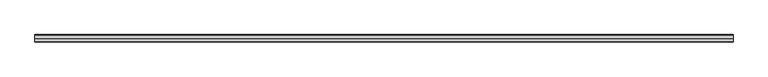
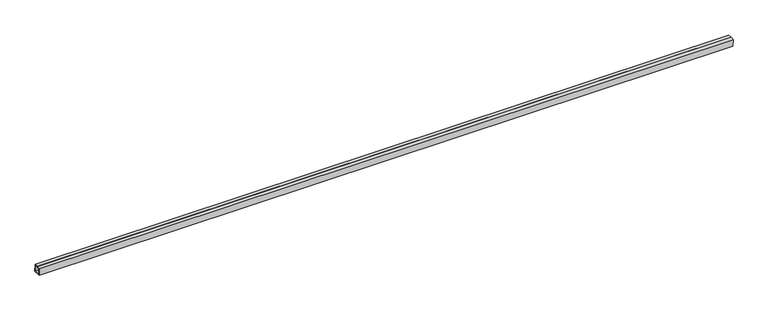
"""IFC4 building model written with IfcOpenShell, lengths in millimetres: proxy geometry, Inner panel:Inner panel:1:Inner panel:1 : Inner panel:Inner panel:300324:2:Inner panel:1:Inner panel:1 : Inner panel:Inner panel:300324:2 : Inner panel:Inner panel:1:Inner panel:1 : Inner panel:Inner panel:300324:300043:19 : Inner panel:Inner panel:1:Inner panel:1 : Inner panel:Inner panel:300324:2:Inner panel:1:Inner panel:1 : Inner panel:Inner panel:300324:2 : Inner panel:Inner panel:1:Inner panel:1 : Inner panel:Inner panel:300324:300043:308120."""

from ifc_helpers import new_model, si_unit, frame, origin, place, context, project, spatial, polyline, outline, extrude, source, transform, mapped, element, save


def generic_models_f3daa5ce(model_context):
    return source(origin(), model_context, "Body", "SweptSolid", [
        extrude(outline(polyline([(-569791.292732, 8736.8354816), (-569773.0523088, 8737.5954993), (-569771.4661851, 8699.5285292), (-569809.5331552, 8697.9424054), (-569811.1192789, 8736.0093755), (-569792.8788557, 8736.7693931), (-569792.779723, 8734.3902075), (-569808.6409605, 8733.7293226), (-569807.2531023, 8700.4207238), (-569773.9445034, 8701.8085821), (-569775.3323617, 8735.1171809), (-569791.1935993, 8734.456296), (-569791.292732, 8736.8354816)])), frame((593141.1867242, 0.0, 0.0), z_axis=(1.0, 0.0, 0.0), x_axis=(0.0, 1.0, 0.0)), (0.0, 0.0, 1.0), 3657.6),
    ])


if __name__ == "__main__":
    model = new_model("IFC4")
    model_context = context("Model", 3, world=origin())
    ifc_project = project(units=[si_unit("LENGTHUNIT", "METRE", prefix="MILLI")], contexts=[model_context])
    site = spatial("IfcSite", under=ifc_project)
    building = spatial("IfcBuilding", under=site)
    placement = place(None, origin())
    generic_models_shape = generic_models_f3daa5ce(model_context)
    element("IfcBuildingElementProxy", 1, Name="Inner panel:Inner panel:1:Inner panel:1 : Inner panel:Inner panel:300324:2:Inner panel:1:Inner panel:1 : Inner panel:Inner panel:300324:2 : Inner panel:Inner panel:1:Inner panel:1 : Inner panel:Inner panel:300324:300043:19 : Inner panel:Inner panel:1:Inner panel:1 : Inner panel:Inner panel:300324:2:Inner panel:1:Inner panel:1 : Inner panel:Inner panel:300324:2 : Inner panel:Inner panel:1:Inner panel:1 : Inner panel:Inner panel:300324:300043:308120", ObjectType="Inner panel:Inner panel:1:Inner panel:1 : Inner panel:Inner panel:300324:2:Inner panel:1:Inner panel:1 : Inner panel:Inner panel:300324:2 : Inner panel:Inner panel:1:Inner panel:1 : Inner panel:Inner panel:300324:300043:19 : Inner panel:Inner panel:1:Inner panel:1 : Inner panel:Inner panel:300324:2:Inner panel:1:Inner panel:1 : Inner panel:Inner panel:300324:2 : Inner panel:Inner panel:1:Inner panel:1 : Inner panel:Inner panel:300324:300043:308120", at=placement, inside=building, context=model_context, shape_type="MappedRepresentation", body=[
        mapped(generic_models_shape, transform((0.0, 0.0, 0.0), x_axis=(1.0, 0.0, 0.0), y_axis=(0.0, 1.0, 0.0), z_axis=(0.0, 0.0, 1.0))),
    ])
    save(model, "model.ifc")

# Revit data of these elements
# Type "Inner panel:Inner panel:1:Inner panel:1 : Inner panel:Inner panel:300324:2:Inner panel:1:Inner panel:1 : Inner panel:Inner panel:300324:2 : Inner panel:Inner panel:1:Inner panel:1 : Inner panel:Inner panel:300324:300043:19 : Inner panel:Inner panel:1:Inner panel:1 : Inner panel:Inner panel:300324:2:Inner panel:1:Inner panel:1 : Inner panel:Inner panel:300324:2 : Inner panel:Inner panel:1:Inner panel:1 : Inner panel:Inner panel:300324:300043:308120"
#   NameOverride = "Inner panel:Inner panel:1:Inner panel:1 : Inner panel:Inner panel:300324:2:Inner panel:1:Inner panel:1 : Inner panel:Inner panel:300324:2 : Inner panel:Inner panel:1:Inner panel:1 : Inner panel:Inner panel:300324:300043:308120"
#   ObjectTypeOverride = "Inner panel:1:Inner panel:1 : Inner panel:Inner panel:300324:2 : Inner panel:Inner panel:1:Inner panel:1 : Inner panel:Inner panel:300324:300043"
#   Reference = "Inner panel"
#   Tag = "308120"
# Element 1 (IfcBuildingElementProxy, "Inner panel:Inner panel:1:Inner panel:1 : Inner panel:Inner panel:300324:2:Inner panel:1:Inner panel:1 : Inner panel:Inner panel:300324:2 : Inner panel:Inner panel:1:Inner panel:1 : Inner panel:Inner panel:300324:300043:19 : Inner panel:Inner panel:1:Inner panel:1 : Inner panel:Inner panel:300324:2:Inner panel:1:Inner panel:1 : Inner panel:Inner panel:300324:2 : Inner panel:Inner panel:1:Inner panel:1 : Inner panel:Inner panel:300324:300043:308120")
#   Materials on its faces: "1 1/2\" X 1 1/2\" SPLIT-SEAM SQUARE TUBING (~24\" CANTILEVER FROM C.L. OF GLULAM)"
# Materials
#   "1 1/2\" X 1 1/2\" SPLIT-SEAM SQUARE TUBING (~24\" CANTILEVER FROM C.L. OF GLULAM)": class "Unassigned", colour RGB 202 201 200, transparency 0, Cost = 0
